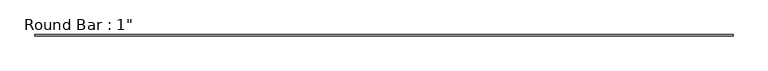
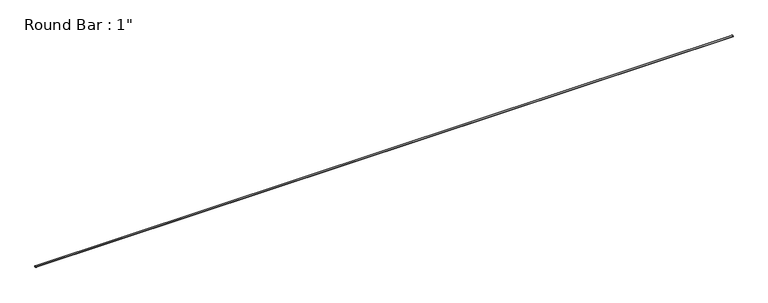
"""IFC4 building model written with IfcOpenShell, lengths in millimetres: member geometry."""

from ifc_helpers import new_model, si_unit, point, frame, origin, origin_2d, place, context, project, spatial, circle_curve, trimmed, segment, composite_curve, outline, extrude, source, transform, mapped, element, save


def member_badfb426(model_context):
    return source(origin(), model_context, "Body", "SweptSolid", [
        extrude(outline(composite_curve([segment(trimmed(circle_curve(origin_2d(), 12.7), [point((-12.7, 0.0))], [point((12.7, 0.0))], False, "CARTESIAN"), True, "CONTINUOUS"), segment(trimmed(circle_curve(origin_2d(), 12.7), [point((12.7, 0.0))], [point((-12.7, 0.0))], False, "CARTESIAN"), True, "CONTINUOUS")], self_intersect=False)), frame((-5592.7009894, 0.0, 0.0), z_axis=(1.0, 0.0, 0.0), x_axis=(0.0, 1.0, 0.0)), (0.0, 0.0, 1.0), 11185.4019788),
    ])


if __name__ == "__main__":
    model = new_model("IFC4")
    model_context = context("Model", 3, world=origin())
    ifc_project = project(units=[si_unit("LENGTHUNIT", "METRE", prefix="MILLI")], contexts=[model_context])
    site = spatial("IfcSite", under=ifc_project)
    building = spatial("IfcBuilding", under=site)
    placement = place(None, origin())
    member_shape = member_badfb426(model_context)
    element("IfcMember", 1, ObjectType="Round Bar : 1\"", at=placement, inside=building, context=model_context, shape_type="MappedRepresentation", body=[
        mapped(member_shape, transform((0.0, 0.0, 0.0), x_axis=(1.0, 0.0, 0.0), y_axis=(0.0, 1.0, 0.0), z_axis=(0.0, 0.0, 1.0))),
    ])
    save(model, "model.ifc")

# Revit data of these elements
# Type "Round Bar : 1\""
#   Assembly Code = "B10"
#   W = 0
#   Start Extension Calculation [instance default] = 10' - 0"
#   Start Extension [instance default] = -0' - 0 1/2"
#   End Extension Calculation [instance default] = 10' - 0"
#   End Extension [instance default] = -0' - 0 1/2"
#   Length [instance default] = 5' - 0"
#   d = 0' - 1"
#   A = 0 SF
#   Structural Material [instance default] = Metal - Steel - ASTM A36
# Element 1 (IfcMember, "Round Bar : 1\"")
#   Materials on its faces: "Metal - Steel - ASTM A36"
# Materials
#   "Metal - Steel - ASTM A36": class "Metal", colour RGB 199 199 199, transparency 0
